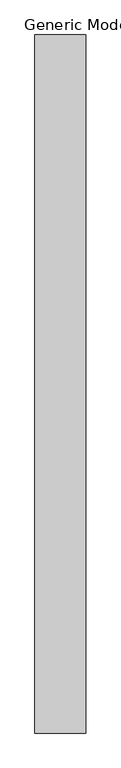
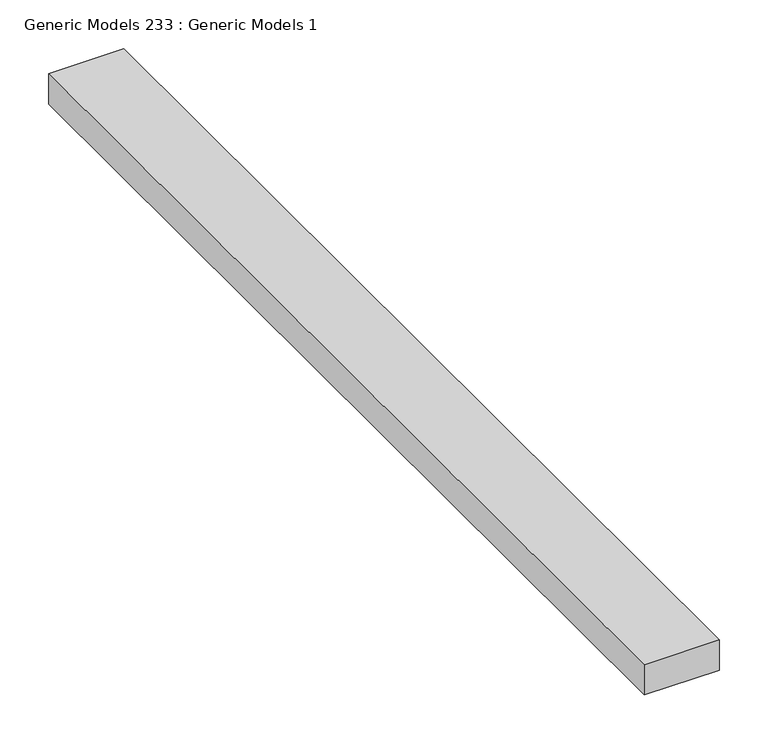
"""IFC4 building model written with IfcOpenShell, lengths in millimetres: proxy geometry, Generic Models 233 : Generic Models 1."""

import ifcopenshell
import ifcopenshell.guid

model = None  # the IFC model being written
_history = None  # IfcOwnerHistory: only IFC2X3 demands one
_inside = {}  # id of a spatial element -> (the spatial element, [elements in it])
_under = {}  # id of a project, library or spatial element -> (it, [spatial elements below it])
_declared = {}  # id of a project -> (the project, [libraries it declares])
_typed = {}  # id of a type object -> (the type object, [elements of that type])
_made_of = {}  # id of a material, layer set ... -> (it, [elements and type objects made of it])


def new_model(schema):
    """Start an empty IFC model of exactly this schema.

    Asked for "IFC4X3", IfcOpenShell would pick the latest addendum, in which some entities
    have other attributes; the version numbers below select the first issue.
    IFC2X3 requires an IfcOwnerHistory on every rooted entity: one is made here for all.
    """
    global model, _history
    if schema == "IFC4X3":
        model = ifcopenshell.file(schema_version=(4, 3, 0, 0))
    else:
        model = ifcopenshell.file(schema=schema)
    _inside.clear()
    _under.clear()
    _declared.clear()
    _typed.clear()
    _made_of.clear()
    _history = None
    if model.schema == "IFC2X3":
        org = make("IfcOrganization", Name="unknown")
        user = make(
            "IfcPersonAndOrganization",
            ThePerson=make("IfcPerson", FamilyName="unknown"),
            TheOrganization=org,
        )
        app = make(
            "IfcApplication",
            ApplicationDeveloper=org,
            Version="unknown",
            ApplicationFullName="unknown",
            ApplicationIdentifier="unknown",
        )
        _history = make(
            "IfcOwnerHistory",
            OwningUser=user,
            OwningApplication=app,
            ChangeAction="ADDED",
            CreationDate=0,
        )
    return model


def make(cls, **values):
    """One entity of the class cls with the attributes given. An attribute that is None is left unset."""
    return model.create_entity(
        cls, **{name: value for name, value in values.items() if value is not None}
    )


def rooted(cls, **values):
    """An entity with a GlobalId (a new one), such as an element, a storey or a relation."""
    return make(cls, GlobalId=ifcopenshell.guid.new(), OwnerHistory=_history, **values)


def si_unit(unit_type, name, prefix=None):
    """IfcSIUnit, for example si_unit("LENGTHUNIT", "METRE", prefix="MILLI")."""
    return make("IfcSIUnit", UnitType=unit_type, Prefix=prefix, Name=name)


def assignment(units):
    """IfcUnitAssignment: the units of a project."""
    return None if units is None else make("IfcUnitAssignment", Units=units)


def point(xyz):
    """IfcCartesianPoint."""
    return None if xyz is None else make("IfcCartesianPoint", Coordinates=xyz)


def direction(xyz):
    """IfcDirection."""
    return None if xyz is None else make("IfcDirection", DirectionRatios=xyz)


def frame(location, z_axis=None, x_axis=None):
    """IfcAxis2Placement3D, a coordinate frame: its origin and axes. An axis left out is left unset."""
    return make(
        "IfcAxis2Placement3D",
        Location=point(location),
        Axis=direction(z_axis),
        RefDirection=direction(x_axis),
    )


def origin():
    """The frame at (0, 0, 0) with its axes left unset."""
    return frame((0.0, 0.0, 0.0))


def place(relative_to, where):
    """IfcLocalPlacement: puts the frame where relative to a parent placement (None: the world)."""
    return make(
        "IfcLocalPlacement", PlacementRelTo=relative_to, RelativePlacement=where
    )


def context(
    kind, dimensions, precision=None, world=None, true_north=None, identifier=None
):
    """IfcGeometricRepresentationContext, for example the 3D "Model" context."""
    return make(
        "IfcGeometricRepresentationContext",
        ContextIdentifier=identifier,
        ContextType=kind,
        CoordinateSpaceDimension=dimensions,
        Precision=precision,
        WorldCoordinateSystem=world,
        TrueNorth=true_north,
    )


def project(units=None, contexts=None):
    """IfcProject with its units and contexts."""
    return rooted(
        "IfcProject",
        Name="project",
        RepresentationContexts=contexts,
        UnitsInContext=assignment(units),
    )


def spatial(cls, under=None, at=None, **own):
    """A site, building, storey or space (cls), placed at a placement, below another one or the project."""
    s = rooted(cls, ObjectPlacement=at, **own)
    if under is not None:
        _under.setdefault(under.id(), (under, []))[1].append(s)
    return s


def polyline(points):
    """IfcPolyline through the points."""
    return make("IfcPolyline", Points=[point(p) for p in points])


def outline(outer, holes=None, kind="AREA"):
    """IfcArbitraryClosedProfileDef: a profile drawn as a closed curve; with holes, ...WithVoids."""
    if holes is None:
        return make("IfcArbitraryClosedProfileDef", ProfileType=kind, OuterCurve=outer)
    return make(
        "IfcArbitraryProfileDefWithVoids",
        ProfileType=kind,
        OuterCurve=outer,
        InnerCurves=holes,
    )


def extrude(swept, where, along, depth):
    """IfcExtrudedAreaSolid: the profile swept, set in the frame where, extruded along a direction by depth."""
    return make(
        "IfcExtrudedAreaSolid",
        SweptArea=swept,
        Position=where,
        ExtrudedDirection=direction(along),
        Depth=depth,
    )


def shape(context_of_items, identifier, shape_type, items):
    """IfcShapeRepresentation: the items that make up one representation, for example the "Body"."""
    return make(
        "IfcShapeRepresentation",
        ContextOfItems=context_of_items,
        RepresentationIdentifier=identifier,
        RepresentationType=shape_type,
        Items=items,
    )


def source(mapping_origin, context_of_items, identifier, shape_type, items):
    """IfcRepresentationMap: a shape defined once, which mapped items show again and again."""
    return make(
        "IfcRepresentationMap",
        MappingOrigin=mapping_origin,
        MappedRepresentation=shape(context_of_items, identifier, shape_type, items),
    )


def transform(
    local_origin,
    x_axis=None,
    y_axis=None,
    z_axis=None,
    scale=None,
    scale2=None,
    scale3=None,
    uniform=True,
):
    """IfcCartesianTransformationOperator3D, or its non-uniform kind. x_axis, y_axis, z_axis: its Axis1, 2, 3."""
    if uniform:
        return make(
            "IfcCartesianTransformationOperator3D",
            Axis1=direction(x_axis),
            Axis2=direction(y_axis),
            LocalOrigin=point(local_origin),
            Scale=scale,
            Axis3=direction(z_axis),
        )
    return make(
        "IfcCartesianTransformationOperator3DnonUniform",
        Axis1=direction(x_axis),
        Axis2=direction(y_axis),
        LocalOrigin=point(local_origin),
        Scale=scale,
        Axis3=direction(z_axis),
        Scale2=scale2,
        Scale3=scale3,
    )


def mapped(mapping_source, mapping_target):
    """IfcMappedItem: shows the shape of a source again, moved by a transform."""
    return make(
        "IfcMappedItem", MappingSource=mapping_source, MappingTarget=mapping_target
    )


def made_of(thing, what):
    """Note that an element or type object is made of a material, layer set ...; save() writes the relation."""
    if what is not None:
        _made_of.setdefault(what.id(), (what, []))[1].append(thing)
    return thing


def element(
    cls,
    number,
    at=None,
    inside=None,
    cuts=None,
    type_object=None,
    material=None,
    context=None,
    identifier="Body",
    shape_type=None,
    held_by="IfcProductDefinitionShape",
    body=None,
    shapes=None,
    **own,
):
    """One element of the class cls, such as IfcWall. Its Tag is "e" and its number.

    at: its placement. inside: the storey or other place that contains it. cuts: it is an
    opening in that element (IfcRelVoidsElement). A single representation is given by context,
    identifier, shape_type and body (its items); several are given by shapes. held_by: the class
    of the entity that holds the representations. save() writes the other relations.
    """
    e = rooted(cls, Tag="e%d" % number, ObjectPlacement=at, **own)
    if body is not None:
        shapes = [shape(context, identifier, shape_type, body)]
    if shapes is not None:
        e.Representation = make(held_by, Representations=shapes)
    if inside is not None:
        _inside.setdefault(inside.id(), (inside, []))[1].append(e)
    if cuts is not None:
        rooted(
            "IfcRelVoidsElement", RelatingBuildingElement=cuts, RelatedOpeningElement=e
        )
    if type_object is not None:
        _typed.setdefault(type_object.id(), (type_object, []))[1].append(e)
    return made_of(e, material)


def aggregate(whole, parts):
    """IfcRelAggregates: a whole, such as a stair, and the parts it consists of."""
    return rooted("IfcRelAggregates", RelatingObject=whole, RelatedObjects=parts)


def save(model, path):
    """Write the relations noted so far, then the file.

    IfcRelAggregates (storeys below a building ...), IfcRelContainedInSpatialStructure (elements
    in a storey), IfcRelDefinesByType, IfcRelAssociatesMaterial and IfcRelDeclares: one each for
    every whole, place, type object, material and project.
    """
    for whole, parts in _under.values():
        aggregate(whole, parts)
    for where, things in _inside.values():
        rooted(
            "IfcRelContainedInSpatialStructure",
            RelatedElements=things,
            RelatingStructure=where,
        )
    for kind, things in _typed.values():
        rooted("IfcRelDefinesByType", RelatedObjects=things, RelatingType=kind)
    for what, things in _made_of.values():
        rooted("IfcRelAssociatesMaterial", RelatedObjects=things, RelatingMaterial=what)
    for by, libraries in _declared.values():
        rooted("IfcRelDeclares", RelatingContext=by, RelatedDefinitions=libraries)
    model.write(path)


def generic_models_233_generic_models_1_ae5bae41(model_context):
    return source(origin(), model_context, "Body", "SweptSolid", [
        extrude(outline(polyline([(48564.8, 0.0), (48475.9, 0.0), (48475.9, 1219.2), (48564.8, 1219.2), (48564.8, 0.0)])), frame((0.0, 0.0, 5467.35), z_axis=(0.0, 0.0, 1.0), x_axis=(1.0, 0.0, 0.0)), (0.0, 0.0, 1.0), 38.1),
    ])


if __name__ == "__main__":
    model = new_model("IFC4")
    model_context = context("Model", 3, world=origin())
    ifc_project = project(units=[si_unit("LENGTHUNIT", "METRE", prefix="MILLI")], contexts=[model_context])
    site = spatial("IfcSite", under=ifc_project)
    building = spatial("IfcBuilding", under=site)
    placement = place(None, origin())
    generic_models_233_generic_models_1_shape = generic_models_233_generic_models_1_ae5bae41(model_context)
    element("IfcBuildingElementProxy", 1, Name="Generic Models 233 : Generic Models 1", ObjectType="Generic Models 233 : Generic Models 1", at=placement, inside=building, context=model_context, shape_type="MappedRepresentation", body=[
        mapped(generic_models_233_generic_models_1_shape, transform((0.0, 0.0, 0.0), x_axis=(1.0, 0.0, 0.0), y_axis=(0.0, 1.0, 0.0), z_axis=(0.0, 0.0, 1.0))),
    ])
    save(model, "model.ifc")

# Revit data of these elements
# Element 1 (IfcBuildingElementProxy, "Generic Models 233 : Generic Models 1")
#   Materials on its faces: "2X WOOD HEADER ATTACHED TO STEEL PURLIN"
# Materials
#   "2X WOOD HEADER ATTACHED TO STEEL PURLIN": class "Wood", colour RGB 234 198 147, transparency 0, Description = "Pinus Echinata", Cost = 0
